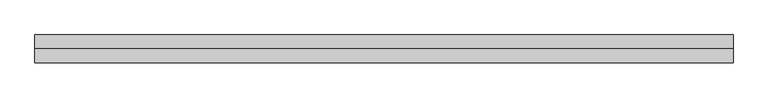
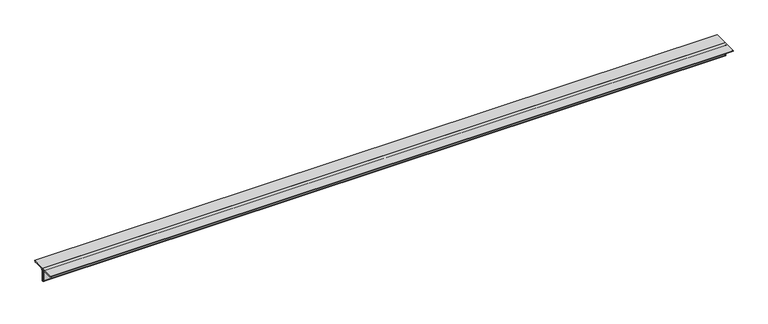
"""IFC4 building model written with IfcOpenShell, lengths in millimetres: member geometry, Steel Framing_2Ls_KS : H_SB_AR_S02_2Ls-100x100x10_VBR1."""

from ifc_helpers import new_model, si_unit, point, frame, frame_2d, origin, place, context, project, spatial, polyline, circle_curve, trimmed, segment, composite_curve, outline, extrude, source, transform, mapped, element, save


def member_75552ef0(model_context):
    return source(origin(), model_context, "Body", "SweptSolid", [
        extrude(outline(composite_curve([segment(polyline([(0.0, 28.2), (0.0, -71.8)]), True, "CONTINUOUS"), segment(trimmed(circle_curve(frame_2d((0.0, -61.8)), 10.0), [point((0.0, -71.8))], [point((-10.0, -61.8))], False, "CARTESIAN"), True, "CONTINUOUS"), segment(polyline([(-10.0, -61.8), (-10.0, 8.2)]), True, "CONTINUOUS"), segment(trimmed(circle_curve(frame_2d((-20.0, 8.2)), 10.0), [point((-10.0, 8.2))], [point((-20.0, 18.2))], True, "CARTESIAN"), True, "CONTINUOUS"), segment(polyline([(-20.0, 18.2), (-90.0, 18.2)]), True, "CONTINUOUS"), segment(trimmed(circle_curve(frame_2d((-90.0, 28.2)), 10.0), [point((-90.0, 18.2))], [point((-100.0, 28.2))], False, "CARTESIAN"), True, "CONTINUOUS"), segment(polyline([(-100.0, 28.2), (0.0, 28.2)]), True, "CONTINUOUS")], self_intersect=False)), frame((-2391.9159074, 0.0, 0.0), z_axis=(1.0, 0.0, 0.0), x_axis=(0.0, 1.0, 0.0)), (0.0, 0.0, 1.0), 4992.4085104),
        extrude(outline(composite_curve([segment(polyline([(0.0, 28.2), (100.0, 28.2)]), True, "CONTINUOUS"), segment(trimmed(circle_curve(frame_2d((90.0, 28.2)), 10.0), [point((100.0, 28.2))], [point((90.0, 18.2))], False, "CARTESIAN"), True, "CONTINUOUS"), segment(polyline([(90.0, 18.2), (20.0, 18.2)]), True, "CONTINUOUS"), segment(trimmed(circle_curve(frame_2d((20.0, 8.2)), 10.0), [point((20.0, 18.2))], [point((10.0, 8.2))], True, "CARTESIAN"), True, "CONTINUOUS"), segment(polyline([(10.0, 8.2), (10.0, -61.8)]), True, "CONTINUOUS"), segment(trimmed(circle_curve(frame_2d((0.0, -61.8)), 10.0), [point((10.0, -61.8))], [point((0.0, -71.8))], False, "CARTESIAN"), True, "CONTINUOUS"), segment(polyline([(0.0, -71.8), (0.0, 28.2)]), True, "CONTINUOUS")], self_intersect=False)), frame((-2391.9159074, 0.0, 0.0), z_axis=(1.0, 0.0, 0.0), x_axis=(0.0, 1.0, 0.0)), (0.0, 0.0, 1.0), 4992.4085104),
    ])


if __name__ == "__main__":
    model = new_model("IFC4")
    model_context = context("Model", 3, world=origin())
    ifc_project = project(units=[si_unit("LENGTHUNIT", "METRE", prefix="MILLI")], contexts=[model_context])
    site = spatial("IfcSite", under=ifc_project)
    building = spatial("IfcBuilding", under=site)
    placement = place(None, origin())
    member_shape = member_75552ef0(model_context)
    element("IfcMember", 1, ObjectType="Steel Framing_2Ls_KS : H_SB_AR_S02_2Ls-100x100x10_VBR1", at=placement, inside=building, context=model_context, shape_type="MappedRepresentation", body=[
        mapped(member_shape, transform((0.0, 0.0, 0.0), x_axis=(1.0, 0.0, 0.0), y_axis=(0.0, 1.0, 0.0), z_axis=(0.0, 0.0, 1.0))),
    ])
    save(model, "model.ifc")

# Revit data of these elements
# Type "Steel Framing_2Ls_KS : H_SB_AR_S02_2Ls-100x100x10_VBR1"
#   Type Comments = "MAIN"
#   Type Mark = "VBR1"
#   H_SectionID = "2Ls-100x100x10"
#   Assembly Code = "B10"
#   Legs = "LLBB"
#   H_Ratio for Additional Steel Plate = 0.2
#   W = 0
#   Perimeter = 0.80 m²/m
#   Nominal Weight = 29.80 kgf/m
#   Length [instance default] = 1524 mm
#   Space = 0 mm
#   b = 100 mm
#   d = 100 mm
#   t = 10 mm
#   y = 28.2 mm
#   A = 0.0038 m²
#   Structural Material [instance default] = Steel, 45-345
# Element 1 (IfcMember, "Steel Framing_2Ls_KS : H_SB_AR_S02_2Ls-100x100x10_VBR1")
#   Materials on its faces: "Steel, 45-345"
# Materials
#   "Steel, 45-345": class "Metal", colour RGB 189 187 185, transparency 0, Description = "Steel 345 MPa", Cost = 0
